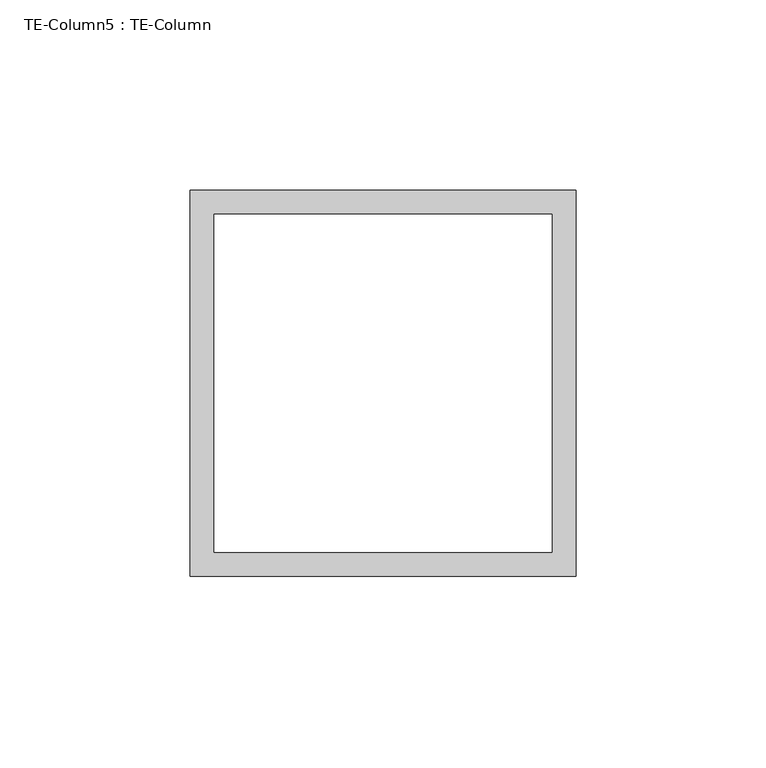
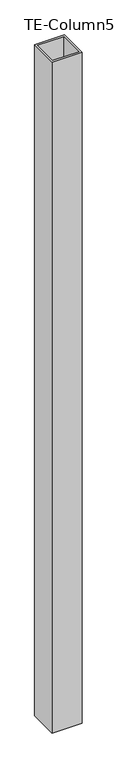
"""IFC4 building model written with IfcOpenShell, lengths in millimetres: proxy geometry, TE-Column5 : TE-Column."""

from ifc_helpers import new_model, si_unit, frame, origin, place, context, project, spatial, polyline, outline, extrude, source, transform, mapped, element, save


def te_column5_te_column_ebccfb0c(model_context):
    return source(origin(), model_context, "Body", "SweptSolid", [
        extrude(outline(polyline([(587468.2808739, -533991.8913841), (587468.2808739, -534093.4913841), (587366.6808739, -534093.4913841), (587366.6808739, -533991.8913841), (587468.2808739, -533991.8913841)]), holes=[polyline([(587373.0308739, -533998.2413841), (587373.0308739, -534087.1413841), (587461.9308739, -534087.1413841), (587461.9308739, -533998.2413841), (587373.0308739, -533998.2413841)])]), frame((0.0, 0.0, 28.575), z_axis=(0.0, 0.0, 1.0), x_axis=(1.0, 0.0, 0.0)), (0.0, 0.0, 1.0), 2406.65),
    ])


if __name__ == "__main__":
    model = new_model("IFC4")
    model_context = context("Model", 3, world=origin())
    ifc_project = project(units=[si_unit("LENGTHUNIT", "METRE", prefix="MILLI")], contexts=[model_context])
    site = spatial("IfcSite", under=ifc_project)
    building = spatial("IfcBuilding", under=site)
    placement = place(None, origin())
    te_column5_te_column_shape = te_column5_te_column_ebccfb0c(model_context)
    element("IfcBuildingElementProxy", 1, Name="TE-Column5 : TE-Column", ObjectType="TE-Column5 : TE-Column", at=placement, inside=building, context=model_context, shape_type="MappedRepresentation", body=[
        mapped(te_column5_te_column_shape, transform((0.0, 0.0, 0.0), x_axis=(1.0, 0.0, 0.0), y_axis=(0.0, 1.0, 0.0), z_axis=(0.0, 0.0, 1.0))),
    ])
    save(model, "model.ifc")

# Revit data of these elements
# Element 1 (IfcBuildingElementProxy, "TE-Column5 : TE-Column")
#   Materials on its faces: "4\"X4\" GALV. HSS TUBING"
# Materials
#   "4\"X4\" GALV. HSS TUBING": class "Generic", colour RGB 211 211 207, transparency 0, Cost = 0
